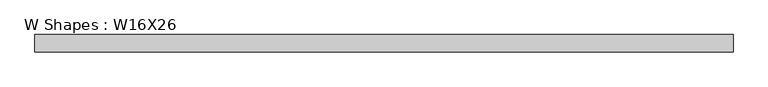
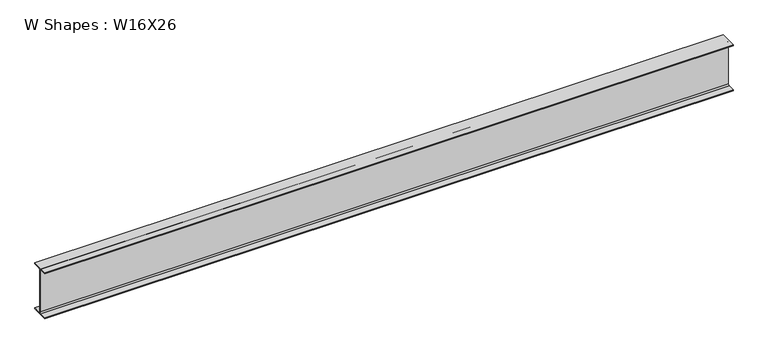
"""IFC4 building model written with IfcOpenShell, lengths in millimetres: beam geometry, W Shapes : W16X26."""

from ifc_helpers import new_model, si_unit, point, frame, frame_2d, origin, place, context, project, spatial, polyline, circle_curve, trimmed, segment, composite_curve, outline, extrude, source, transform, mapped, element, save


def w_shapes_w16x26_33867d62(model_context):
    return source(origin(), model_context, "Body", "SweptSolid", [
        extrude(outline(composite_curve([segment(polyline([(69.85, -190.627), (69.85, -199.39), (-69.85, -199.39), (-69.85, -190.627), (-13.3858, -190.627)]), True, "CONTINUOUS"), segment(trimmed(circle_curve(frame_2d((-13.3858, -180.4162)), 10.2108), [point((-13.3858, -190.627))], [point((-3.175, -180.4162))], True, "CARTESIAN"), True, "CONTINUOUS"), segment(polyline([(-3.175, -180.4162), (-3.175, 180.4162)]), True, "CONTINUOUS"), segment(trimmed(circle_curve(frame_2d((-13.3858, 180.4162)), 10.2108), [point((-3.175, 180.4162))], [point((-13.3858, 190.627))], True, "CARTESIAN"), True, "CONTINUOUS"), segment(polyline([(-13.3858, 190.627), (-69.85, 190.627), (-69.85, 199.39), (69.85, 199.39), (69.85, 190.627), (13.3858, 190.627)]), True, "CONTINUOUS"), segment(trimmed(circle_curve(frame_2d((13.3858, 180.4162)), 10.2108), [point((13.3858, 190.627))], [point((3.175, 180.4162))], True, "CARTESIAN"), True, "CONTINUOUS"), segment(polyline([(3.175, 180.4162), (3.175, -180.4162)]), True, "CONTINUOUS"), segment(trimmed(circle_curve(frame_2d((13.3858, -180.4162)), 10.2108), [point((3.175, -180.4162))], [point((13.3858, -190.627))], True, "CARTESIAN"), True, "CONTINUOUS"), segment(polyline([(13.3858, -190.627), (69.85, -190.627)]), True, "CONTINUOUS")], self_intersect=False)), frame((-2819.4, 0.0, 0.0), z_axis=(1.0, 0.0, 0.0), x_axis=(0.0, 1.0, 0.0)), (0.0, 0.0, 1.0), 5638.8),
    ])


if __name__ == "__main__":
    model = new_model("IFC4")
    model_context = context("Model", 3, world=origin())
    ifc_project = project(units=[si_unit("LENGTHUNIT", "METRE", prefix="MILLI")], contexts=[model_context])
    site = spatial("IfcSite", under=ifc_project)
    building = spatial("IfcBuilding", under=site)
    placement = place(None, origin())
    w_shapes_w16x26_shape = w_shapes_w16x26_33867d62(model_context)
    element("IfcBeam", 1, ObjectType="W Shapes : W16X26", at=placement, inside=building, context=model_context, shape_type="MappedRepresentation", body=[
        mapped(w_shapes_w16x26_shape, transform((0.0, 0.0, 0.0), x_axis=(1.0, 0.0, 0.0), y_axis=(0.0, 1.0, 0.0), z_axis=(0.0, 0.0, 1.0))),
    ])
    save(model, "model.ifc")

# Revit data of these elements
# Type "W Shapes : W16X26"
#   Section Name Key = "W16x26"
#   Assembly Code = "B10"
#   Width = 5.500"
#   Web Thickness = 0.250"
#   Web Fillet = 0.402"
#   Warping Constant = 565.00 in⁶
#   Torsional Moment of Inertia = 0.262 in⁴
#   Section Area = 7.68 in²
#   Plastic Modulus weak axis = 5.48 in³
#   Plastic Modulus strong axis = 44.20 in³
#   Perimeter = 4.35 ft²/ft
#   Nominal Weight = 26.00 lbf/ft
#   Moment of Inertia weak axis = 9.59 in⁴
#   Moment of Inertia strong axis = 301.00 in⁴
#   Height = 15.700"
#   Flange Thickness = 0.345"
#   Elastic Modulus weak axis = 3.49 in³
#   Elastic Modulus strong axis = 38.40 in³
#   Centroid Vertical = 7.850"
#   Centroid Horizontal = 2.750"
#   Bolt Spacing = 0' - 3 1/2"
#   Length [instance default] = 5' - 0"
#   Structural Material [instance default] = Steel ASTM A992
#   Principal Axes Angle = 0
# Element 1 (IfcBeam, "W Shapes : W16X26")
#   Structural Material = Steel ASTM A36
#   Materials on its faces: "Steel ASTM A36"
# Materials
#   "Steel ASTM A992": class "Metal", colour RGB 199 199 199, transparency 0, Description = "Structural steel 50ksi", Cost = 0
#   "Steel ASTM A36": class "Metal", colour RGB 199 199 199, transparency 0, Description = "Structural steel, ASTM A36 Grade B, mill finish", Cost = 0
